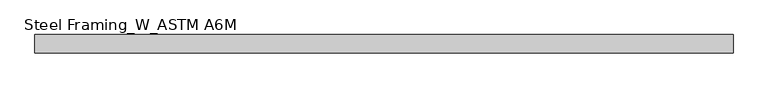
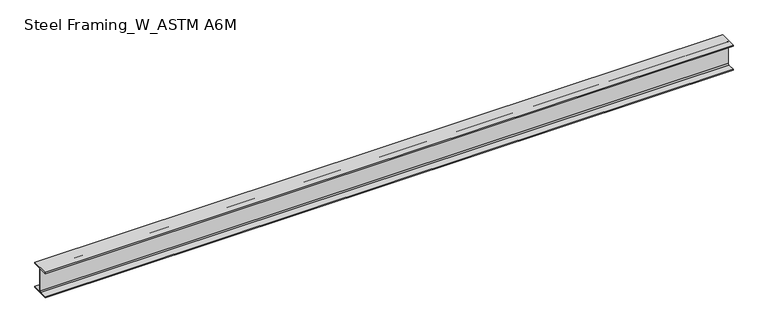
"""IFC4 building model written with IfcOpenShell, lengths in millimetres: beam geometry, Steel Framing_W_ASTM A6M : H_SB_AR_S02_W310x60_B5."""

from ifc_helpers import new_model, si_unit, point, frame, frame_2d, origin, place, context, project, spatial, polyline, circle_curve, trimmed, segment, composite_curve, outline, extrude, source, transform, mapped, element, save


def steel_framing_w_astm_a6m_441ca15e(model_context):
    return source(origin(), model_context, "Body", "SweptSolid", [
        extrude(outline(composite_curve([segment(polyline([(101.5, -137.9), (101.5, -151.0), (-101.5, -151.0), (-101.5, -137.9), (-16.545, -137.9)]), True, "CONTINUOUS"), segment(trimmed(circle_curve(frame_2d((-16.545, -125.1)), 12.8), [point((-16.545, -137.9))], [point((-3.745, -125.1))], True, "CARTESIAN"), True, "CONTINUOUS"), segment(polyline([(-3.745, -125.1), (-3.745, 125.1)]), True, "CONTINUOUS"), segment(trimmed(circle_curve(frame_2d((-16.545, 125.1)), 12.8), [point((-3.745, 125.1))], [point((-16.545, 137.9))], True, "CARTESIAN"), True, "CONTINUOUS"), segment(polyline([(-16.545, 137.9), (-101.5, 137.9), (-101.5, 151.0), (101.5, 151.0), (101.5, 137.9), (16.545, 137.9)]), True, "CONTINUOUS"), segment(trimmed(circle_curve(frame_2d((16.545, 125.1)), 12.8), [point((16.545, 137.9))], [point((3.745, 125.1))], True, "CARTESIAN"), True, "CONTINUOUS"), segment(polyline([(3.745, 125.1), (3.745, -125.1)]), True, "CONTINUOUS"), segment(trimmed(circle_curve(frame_2d((16.545, -125.1)), 12.8), [point((3.745, -125.1))], [point((16.545, -137.9))], True, "CARTESIAN"), True, "CONTINUOUS"), segment(polyline([(16.545, -137.9), (101.5, -137.9)]), True, "CONTINUOUS")], self_intersect=False)), frame((-3885.8, 0.0, 0.0), z_axis=(1.0, 0.0, 0.0), x_axis=(0.0, 1.0, 0.0)), (0.0, 0.0, 1.0), 7771.6),
    ])


if __name__ == "__main__":
    model = new_model("IFC4")
    model_context = context("Model", 3, world=origin())
    ifc_project = project(units=[si_unit("LENGTHUNIT", "METRE", prefix="MILLI")], contexts=[model_context])
    site = spatial("IfcSite", under=ifc_project)
    building = spatial("IfcBuilding", under=site)
    placement = place(None, origin())
    steel_framing_w_astm_a6m_shape = steel_framing_w_astm_a6m_441ca15e(model_context)
    element("IfcBeam", 1, ObjectType="Steel Framing_W_ASTM A6M : H_SB_AR_S02_W310x60_B5", at=placement, inside=building, context=model_context, shape_type="MappedRepresentation", body=[
        mapped(steel_framing_w_astm_a6m_shape, transform((0.0, 0.0, 0.0), x_axis=(1.0, 0.0, 0.0), y_axis=(0.0, 1.0, 0.0), z_axis=(0.0, 0.0, 1.0))),
    ])
    save(model, "model.ifc")

# Revit data of these elements
# Type "Steel Framing_W_ASTM A6M : H_SB_AR_S02_W310x60_B5"
#   Type Mark = "B5"
#   Section Name Key = "W12x40"
#   Width = 20.3 cm
#   Web Thickness = 0.749 cm
#   Web Fillet = 1.28 cm
#   Warping Constant = 387000.0 cm⁶
#   Torsional Moment of Inertia = 37.70 cm⁴
#   Section Area = 75.5 cm²
#   Plastic Modulus weak axis = 275.0 cm³
#   Plastic Modulus strong axis = 934.0 cm³
#   Perimeter = 1.38 m²/m
#   Nominal Weight = 60.00 kgf/m
#   Moment of Inertia weak axis = 1840.00 cm⁴
#   Moment of Inertia strong axis = 12800.00 cm⁴
#   Height = 30.2 cm
#   Flange Thickness = 1.31 cm
#   Elastic Modulus weak axis = 180.0 cm³
#   Elastic Modulus strong axis = 844.0 cm³
#   Centroid Vertical = 15.1 cm
#   Centroid Horizontal = 10.15 cm
#   Length [instance default] = 1500 mm
#   Structural Material [instance default] = Steel, 45-345
#   Bolt Spacing = 0
#   Assembly Code = ""
# Element 1 (IfcBeam, "Steel Framing_W_ASTM A6M : H_SB_AR_S02_W310x60_B5")
#   Materials on its faces: "Steel, 45-345"
# Materials
#   "Steel, 45-345": class "Metal", colour RGB 189 187 185, transparency 0, Description = "Steel 345 MPa", Cost = 0
